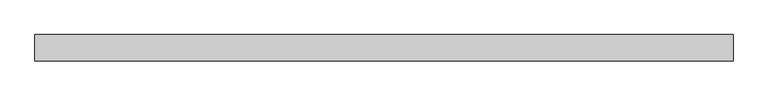
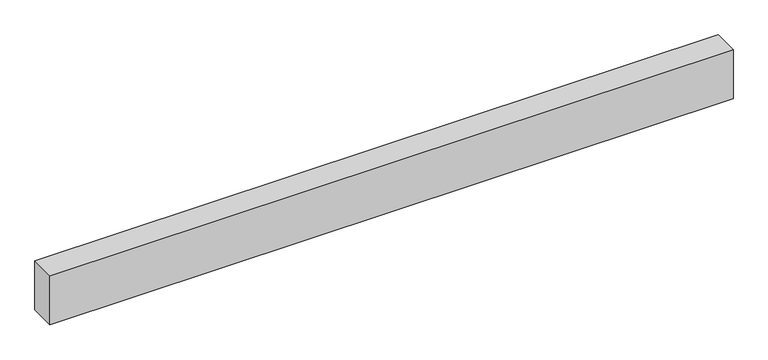
"""IFC4 building model written with IfcOpenShell, lengths in millimetres: beam geometry, Madeira de lei : Berço 6x12cm."""

from ifc_helpers import new_model, si_unit, frame, origin, place, context, project, spatial, polyline, outline, extrude, source, transform, mapped, element, save


def beam_531541e1(model_context):
    return source(origin(), model_context, "Body", "SweptSolid", [
        extrude(outline(polyline([(789.5608169, 30.0), (789.5608169, -30.0), (-789.5608169, -30.0), (-789.5608169, 30.0), (789.5608169, 30.0)])), frame((0.0, 0.0, -60.0), z_axis=(0.0, 0.0, 1.0), x_axis=(1.0, 0.0, 0.0)), (0.0, 0.0, 1.0), 120.0),
    ])


if __name__ == "__main__":
    model = new_model("IFC4")
    model_context = context("Model", 3, world=origin())
    ifc_project = project(units=[si_unit("LENGTHUNIT", "METRE", prefix="MILLI")], contexts=[model_context])
    site = spatial("IfcSite", under=ifc_project)
    building = spatial("IfcBuilding", under=site)
    placement = place(None, origin())
    beam_shape = beam_531541e1(model_context)
    element("IfcBeam", 1, ObjectType="Madeira de lei : Berço 6x12cm", at=placement, inside=building, context=model_context, shape_type="MappedRepresentation", body=[
        mapped(beam_shape, transform((0.0, 0.0, 0.0), x_axis=(1.0, 0.0, 0.0), y_axis=(0.0, 1.0, 0.0), z_axis=(0.0, 0.0, 1.0))),
    ])
    save(model, "model.ifc")

# Revit data of these elements
# Type "Madeira de lei : Berço 6x12cm"
#   A = 0.02 m²
#   Length [instance default] = 1.524 m
#   b = 0.06 m
#   d = 0.12 m
#   Structural Material [instance default] = none
#   Assembly Code = ""
# Element 1 (IfcBeam, "Madeira de lei : Berço 6x12cm")
#   Structural Material = .MADEIRAMENTO
#   Materials on its faces: ".MADEIRAMENTO"
# Materials
#   ".MADEIRAMENTO": class ".CC_MADEIRAS", colour RGB 212 179 113, transparency 0, Cost = 0
